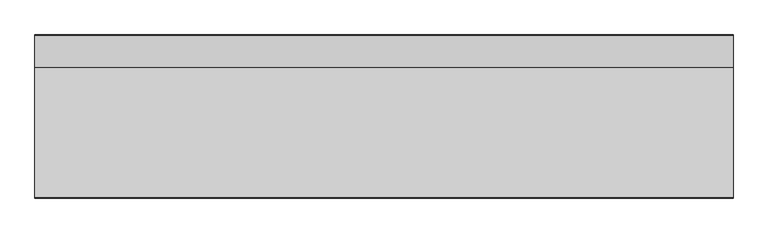
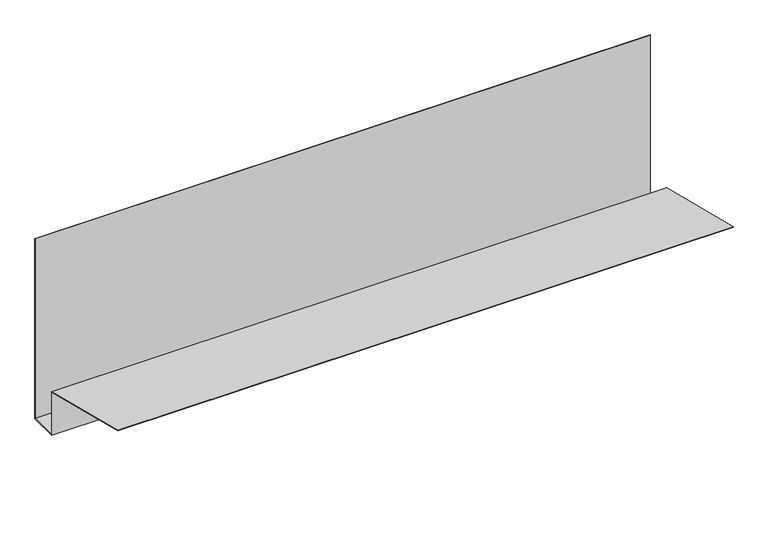
"""IFC4 building model written with IfcOpenShell, lengths in millimetres: proxy geometry, Gutter Adherance Membrane001 : Gutter Adherance Membrane001."""

from ifc_helpers import new_model, si_unit, frame, origin, place, context, project, spatial, polyline, outline, extrude, source, transform, mapped, element, save


def generic_models_a0e20604(model_context):
    return source(origin(), model_context, "Body", "SweptSolid", [
        extrude(outline(polyline([(3992.0115015, 41585.6613751), (4364.6724608, 41492.681487), (4364.6724608, 41344.7151778), (4457.26134, 41344.7151778), (4457.26134, 41961.4921875), (4458.84884, 41961.4921875), (4458.84884, 41343.1276778), (4363.0849609, 41343.1276778), (4363.0849609, 41491.4414062), (3991.6271973, 41584.1210937), (3992.0115015, 41585.6613751)])), frame((255.0171875, 0.0, 0.0), z_axis=(1.0, 0.0, 0.0), x_axis=(0.0, 1.0, 0.0)), (0.0, 0.0, 1.0), 1999.85),
    ])


if __name__ == "__main__":
    model = new_model("IFC4")
    model_context = context("Model", 3, world=origin())
    ifc_project = project(units=[si_unit("LENGTHUNIT", "METRE", prefix="MILLI")], contexts=[model_context])
    site = spatial("IfcSite", under=ifc_project)
    building = spatial("IfcBuilding", under=site)
    placement = place(None, origin())
    generic_models_shape = generic_models_a0e20604(model_context)
    element("IfcBuildingElementProxy", 1, Name="Gutter Adherance Membrane001 : Gutter Adherance Membrane001", ObjectType="Gutter Adherance Membrane001 : Gutter Adherance Membrane001", at=placement, inside=building, context=model_context, shape_type="MappedRepresentation", body=[
        mapped(generic_models_shape, transform((0.0, 0.0, 0.0), x_axis=(1.0, 0.0, 0.0), y_axis=(0.0, 1.0, 0.0), z_axis=(0.0, 0.0, 1.0))),
    ])
    save(model, "model.ifc")

# Revit data of these elements
# Type "Gutter Adherance Membrane001 : Gutter Adherance Membrane001"
#   NameOverride = "Gutter Adherance Membrane001"
# Element 1 (IfcBuildingElementProxy, "Gutter Adherance Membrane001 : Gutter Adherance Membrane001")
#   Materials on its faces: "SELF ADHERED MEMBRANE W/ END DAMS WHERE POSSIBLE"
# Materials
#   "SELF ADHERED MEMBRANE W/ END DAMS WHERE POSSIBLE": class "Unassigned", colour RGB 255 255 127, transparency 0
